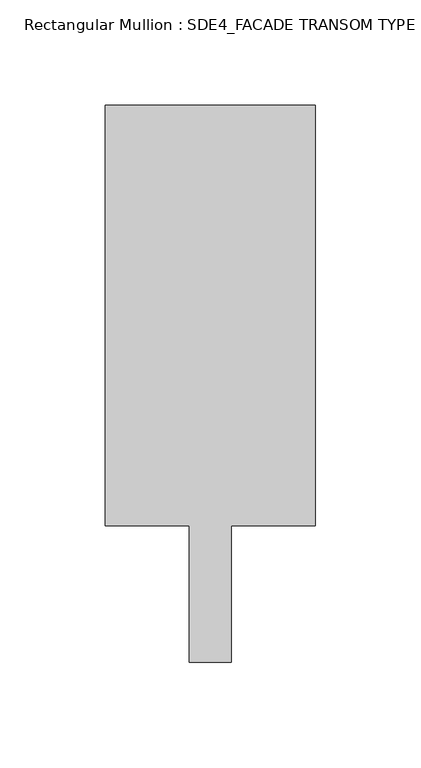
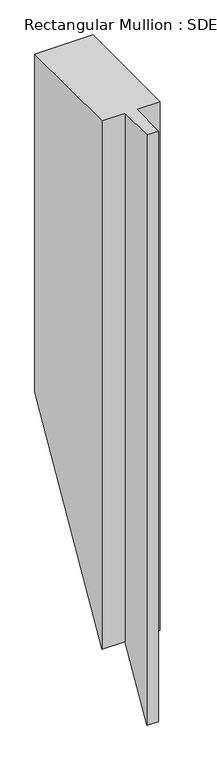
"""IFC4 building model written with IfcOpenShell, lengths in millimetres: member geometry, Rectangular Mullion : SDE4_FACADE TRANSOM TYPE 2."""

from ifc_helpers import new_model, si_unit, origin, place, context, project, spatial, faceted_brep, source, transform, mapped, element, save


def rectangular_mullion_sde4_facade_transom_type_2_1b188930(model_context):
    return source(origin(), model_context, "Body", "Brep", [
        faceted_brep([(50.0, 132.5, 0.0), (-50.0, 132.5, 0.0), (-50.0, -67.5, 0.0), (-10.0, -67.5, 0.0), (-10.0, -132.5, 0.0), (10.0, -132.5, 0.0), (10.0, -67.5, 0.0), (50.0, -67.5, 0.0), (50.0, 132.5, -613.4501572), (-50.0, 132.5, -613.4501572), (-50.0, -67.5, -960.1447994), (-10.0, -67.5, -960.1447994), (-10.0, -132.5, -1072.8205581), (10.0, -132.5, -1072.8205581), (10.0, -67.5, -960.1447994), (50.0, -67.5, -960.1447994)], [[[0, 1, 2, 3, 4, 5, 6, 7]], [[1, 0, 8, 9]], [[2, 1, 9, 10]], [[3, 2, 10, 11]], [[4, 3, 11, 12]], [[5, 4, 12, 13]], [[6, 5, 13, 14]], [[7, 6, 14, 15]], [[0, 7, 15, 8]], [[8, 15, 14, 13, 12, 11, 10, 9]]]),
    ])


if __name__ == "__main__":
    model = new_model("IFC4")
    model_context = context("Model", 3, world=origin())
    ifc_project = project(units=[si_unit("LENGTHUNIT", "METRE", prefix="MILLI")], contexts=[model_context])
    site = spatial("IfcSite", under=ifc_project)
    building = spatial("IfcBuilding", under=site)
    placement = place(None, origin())
    rectangular_mullion_sde4_facade_transom_type_2_shape = rectangular_mullion_sde4_facade_transom_type_2_1b188930(model_context)
    element("IfcMember", 1, ObjectType="Rectangular Mullion : SDE4_FACADE TRANSOM TYPE 2", at=placement, inside=building, context=model_context, shape_type="MappedRepresentation", body=[
        mapped(rectangular_mullion_sde4_facade_transom_type_2_shape, transform((0.0, 0.0, 0.0), x_axis=(1.0, 0.0, 0.0), y_axis=(0.0, 1.0, 0.0), z_axis=(0.0, 0.0, 1.0))),
    ])
    save(model, "model.ifc")

# Revit data of these elements
# Type "Rectangular Mullion : SDE4_FACADE TRANSOM TYPE 2"
#   built-in parameter 1007322 = 0.869423 (stored number, unit not read)
#   built-in parameter 1007321 = 0.164042 (stored number, unit not read)
#   built-in parameter 1007320 = 0.164042 (stored number, unit not read)
